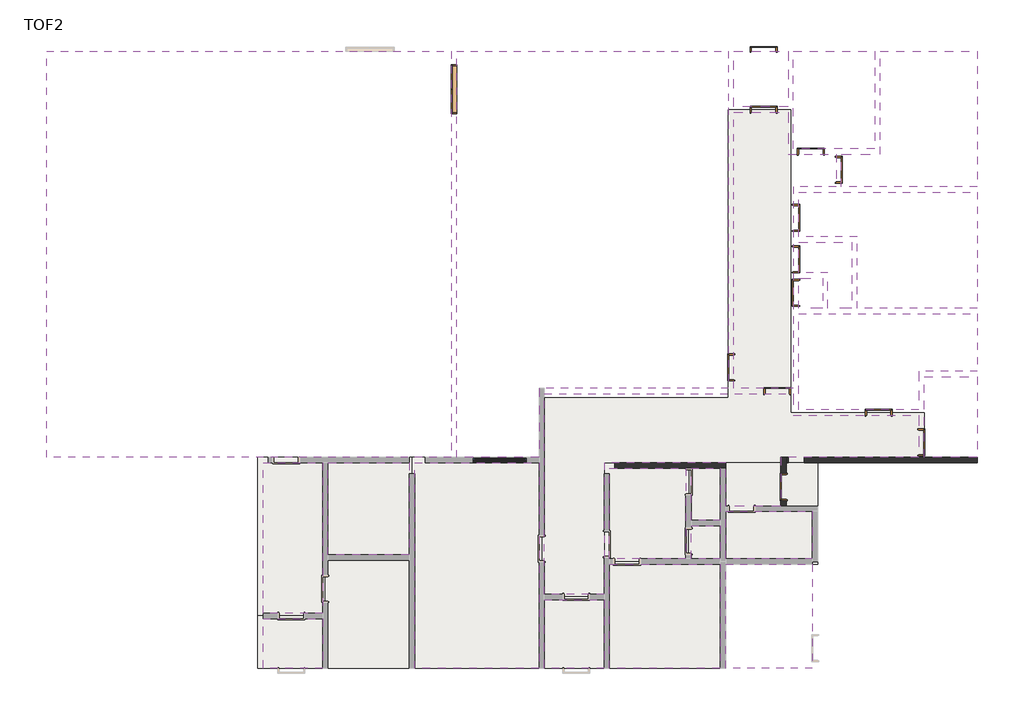
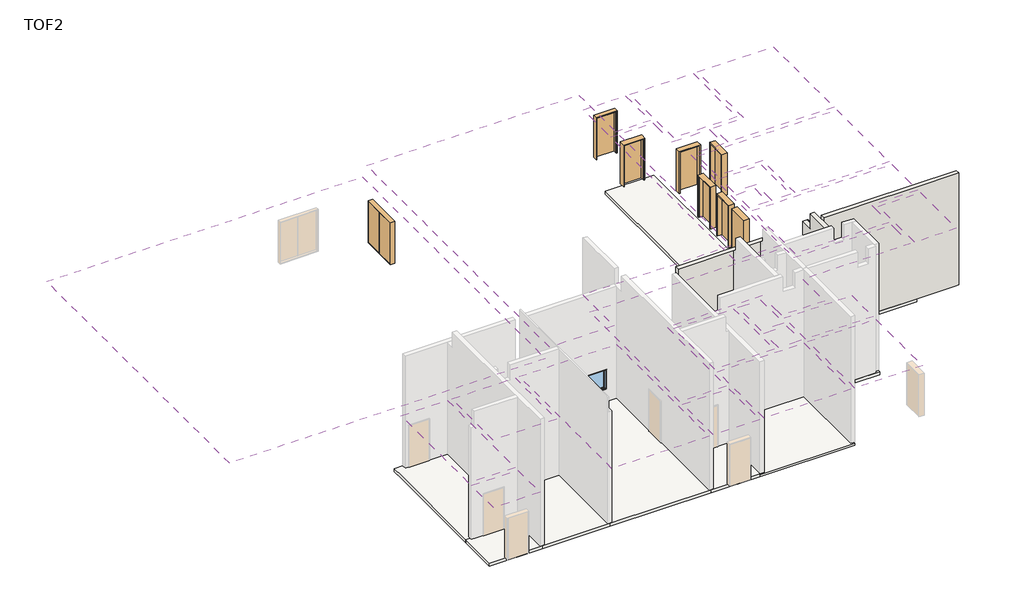
# One storey, part 2 of 2: 23 coverings, 13 doors, 12 slabs, 3 walls, 1 window.
# Revit data of these elements (continued)
# Elements 49, 50, 51 (IfcWall, "H_WA_AR_B02_Int Wall_Block T200") (continued)
#   H_Wall_Finish-In = "Acrylic Emulsion Paint on Cement Plaster"
#   H_Wall_Base Material-3 = ""
#   H_Wall_Finish-Ex = "Acrylic Emulsion Paint on Cement Plaster"
#   H_Wall_Style Remark = "WM : Reinforced Concrete Block\n     50mm<THK≤100mm / 100mm<THK≤200mm / 200mm<THK"
#   Top Offset = 0 mm
#   Base Offset = 0 mm
#   wall height = 6500 mm
#   H_Wall Style No = IW21
#   Phase Created = New Construction
#   Base Constraint = TOF2
#   Top Constraint = TOC
#   Materials on its faces: "00_Masonry_Conc. Block"
# Element 52 (IfcWindow, "Sliding Window : H_WD_AR_B11_Sliding_Steel Window_DG_W2000xH1000")
#   Mark = "FRW-01"
#   H_Window Style Name = "Steel Window_DG_Comb"
#   H_Window_Glass = "Double Glazing"
#   H_Window_Frame = "Steel"
#   H_Window_Fire Rating = "NA/0.5/1.0"
#   H_Window_Style Remark = ""
#   H_Window Style No = WN42
#   Phase Created = New Construction
# Materials
#   "Concrete - Cast-in-Place Concrete - 35 MPa": class "Concrete", colour RGB 192 192 192, transparency 0, Cost = 0
#   "00_Masonry_Conc. Block": class "Concrete", colour RGB 180 180 180, transparency 0, Description = "Conc. Block", Cost = 0, Image = Brick_Uniform_12inch_Running_Gray.png
